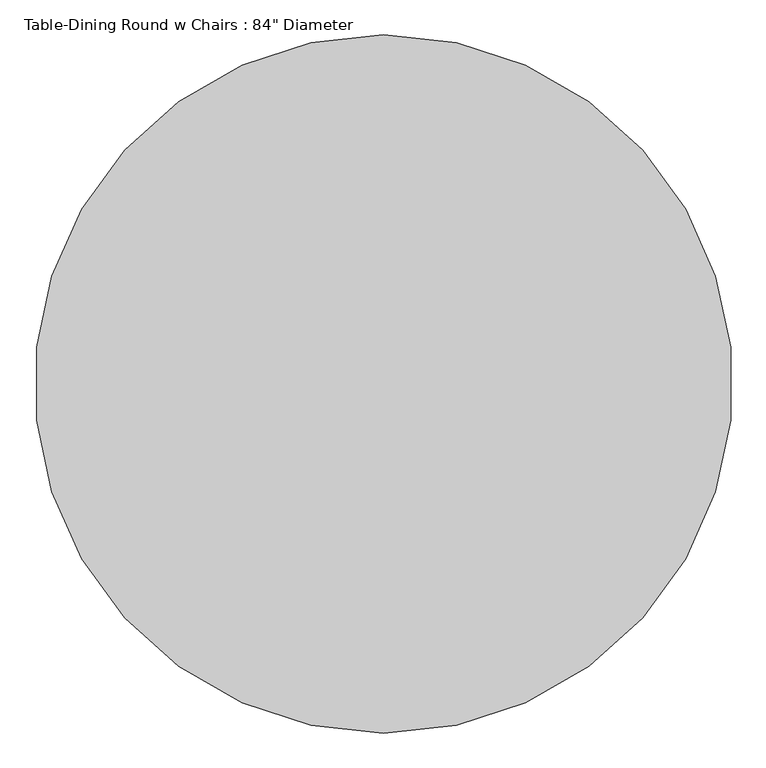
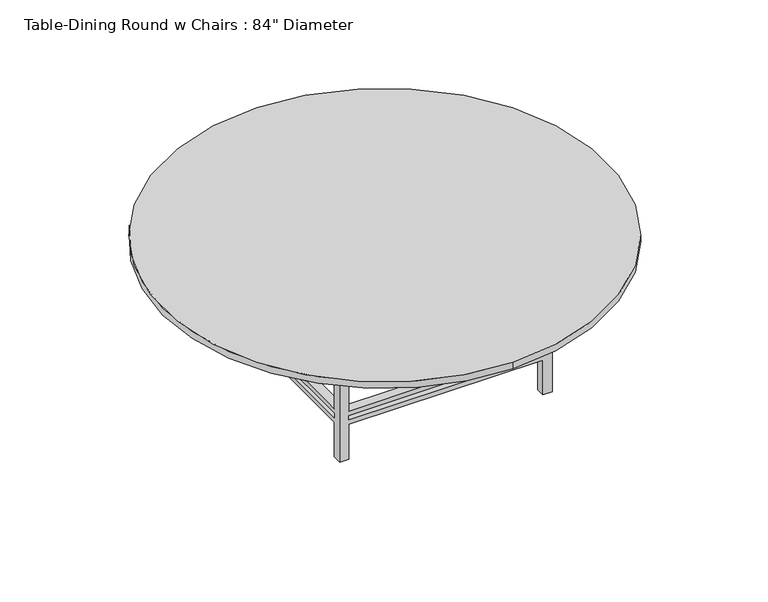
"""IFC4 building model written with IfcOpenShell, lengths in millimetres: furniture geometry."""

from ifc_helpers import new_model, si_unit, point, frame, frame_2d, origin, place, context, project, spatial, polyline, circle_curve, trimmed, segment, composite_curve, outline, extrude, faceted_brep, source, transform, mapped, element, save


def furniture_9698bf4d(model_context):
    return source(origin(), model_context, "Body", "SolidModel", [
        extrude(outline(polyline([(713.2819672, 424.7213115), (713.2819672, -794.4786885), (-505.9180328, -794.4786885), (-505.9180328, 424.7213115), (713.2819672, 424.7213115)]), holes=[polyline([(687.8819672, 399.3213115), (-480.5180328, 399.3213115), (-480.5180328, -769.0786885), (687.8819672, -769.0786885), (687.8819672, 399.3213115)])]), frame((0.0, 0.0, 647.7), z_axis=(0.0, 0.0, 1.0), x_axis=(1.0, 0.0, 0.0)), (0.0, 0.0, 1.0), 76.2),
        faceted_brep([(637.0819672, 348.5213115, 279.4), (637.0819672, -718.2786885, 279.4), (687.8819672, -718.2786885, 279.4), (687.8819672, 348.5213115, 279.4), (-429.7180328, -718.2786885, 279.4), (-429.7180328, -769.0786885, 279.4), (637.0819672, -769.0786885, 279.4), (-429.7180328, 348.5213115, 279.4), (-480.5180328, 348.5213115, 279.4), (-480.5180328, -718.2786885, 279.4), (637.0819672, 399.3213115, 279.4), (-429.7180328, 399.3213115, 279.4), (637.0819672, 348.5213115, 254.0), (-429.7180328, 348.5213115, 254.0), (-429.7180328, 399.3213115, 254.0), (637.0819672, 399.3213115, 254.0), (-429.7180328, -718.2786885, 254.0), (-480.5180328, -718.2786885, 254.0), (-480.5180328, 348.5213115, 254.0), (637.0819672, -718.2786885, 254.0), (637.0819672, -769.0786885, 254.0), (-429.7180328, -769.0786885, 254.0), (687.8819672, 348.5213115, 254.0), (687.8819672, -718.2786885, 254.0), (-480.5180328, 399.3213115, 647.7), (-429.7180328, 399.3213115, 647.7), (637.0819672, 399.3213115, 647.7), (687.8819672, 399.3213115, 647.7), (687.8819672, 399.3213115, 0.0), (637.0819672, 399.3213115, 0.0), (637.0819672, 399.3213115, 203.2), (-429.7180328, 399.3213115, 203.2), (-429.7180328, 399.3213115, 0.0), (-480.5180328, 399.3213115, 0.0), (-429.7180328, 399.3213115, 228.6), (637.0819672, 399.3213115, 228.6), (-480.5180328, 348.5213115, 647.7), (-480.5180328, 348.5213115, 0.0), (-480.5180328, 348.5213115, 203.2), (-480.5180328, -718.2786885, 203.2), (-480.5180328, -718.2786885, 0.0), (-480.5180328, -769.0786885, 0.0), (-480.5180328, -769.0786885, 647.7), (-480.5180328, -718.2786885, 647.7), (-480.5180328, -718.2786885, 228.6), (-480.5180328, 348.5213115, 228.6), (687.8819672, -769.0786885, 647.7), (637.0819672, -769.0786885, 647.7), (-429.7180328, -769.0786885, 647.7), (-429.7180328, -769.0786885, 0.0), (-429.7180328, -769.0786885, 203.2), (637.0819672, -769.0786885, 203.2), (637.0819672, -769.0786885, 0.0), (687.8819672, -769.0786885, 0.0), (637.0819672, -769.0786885, 228.6), (-429.7180328, -769.0786885, 228.6), (687.8819672, 348.5213115, 647.7), (687.8819672, -718.2786885, 647.7), (687.8819672, -718.2786885, 0.0), (687.8819672, -718.2786885, 203.2), (687.8819672, 348.5213115, 203.2), (687.8819672, 348.5213115, 0.0), (687.8819672, 348.5213115, 228.6), (687.8819672, -718.2786885, 228.6), (-429.7180328, 348.5213115, 647.7), (637.0819672, -718.2786885, 647.7), (637.0819672, 348.5213115, 647.7), (-429.7180328, -718.2786885, 647.7), (637.0819672, 348.5213115, 0.0), (-429.7180328, -718.2786885, 0.0), (-429.7180328, 348.5213115, 0.0), (637.0819672, -718.2786885, 0.0), (-429.7180328, 348.5213115, 228.6), (-429.7180328, 348.5213115, 203.2), (637.0819672, 348.5213115, 228.6), (637.0819672, 348.5213115, 203.2), (637.0819672, -718.2786885, 228.6), (637.0819672, -718.2786885, 203.2), (-429.7180328, -718.2786885, 228.6), (-429.7180328, -718.2786885, 203.2)], [[[0, 1, 2, 3]], [[1, 4, 5, 6]], [[4, 7, 8, 9]], [[7, 0, 10, 11]], [[12, 13, 14, 15]], [[13, 16, 17, 18]], [[16, 19, 20, 21]], [[19, 12, 22, 23]], [[24, 25, 11, 10, 26, 27, 28, 29, 30, 31, 32, 33], [14, 34, 35, 15]], [[36, 24, 33, 37, 38, 39, 40, 41, 42, 43, 9, 8], [17, 44, 45, 18]], [[46, 47, 6, 5, 48, 42, 41, 49, 50, 51, 52, 53], [20, 54, 55, 21]], [[28, 27, 56, 3, 2, 57, 46, 53, 58, 59, 60, 61], [22, 62, 63, 23]], [[1, 0, 12, 19]], [[4, 1, 19, 16]], [[7, 4, 16, 13]], [[0, 7, 13, 12]], [[25, 24, 36, 64]], [[47, 46, 57, 65]], [[26, 66, 56, 27]], [[48, 67, 43, 42]], [[29, 28, 61, 68]], [[49, 41, 40, 69]], [[32, 70, 37, 33]], [[52, 71, 58, 53]], [[13, 18, 45, 72]], [[64, 36, 8, 7]], [[37, 70, 73, 38]], [[14, 13, 72, 34]], [[25, 64, 7, 11]], [[70, 32, 31, 73]], [[12, 15, 35, 74]], [[66, 26, 10, 0]], [[29, 68, 75, 30]], [[22, 12, 74, 62]], [[56, 66, 0, 3]], [[68, 61, 60, 75]], [[19, 23, 63, 76]], [[65, 57, 2, 1]], [[58, 71, 77, 59]], [[20, 19, 76, 54]], [[47, 65, 1, 6]], [[71, 52, 51, 77]], [[16, 21, 55, 78]], [[67, 48, 5, 4]], [[49, 69, 79, 50]], [[17, 16, 78, 44]], [[43, 67, 4, 9]], [[69, 40, 39, 79]], [[74, 76, 63, 62]], [[76, 78, 55, 54]], [[78, 72, 45, 44]], [[72, 74, 35, 34]], [[75, 73, 31, 30]], [[73, 79, 39, 38]], [[79, 77, 51, 50]], [[77, 75, 60, 59]], [[76, 74, 75, 77]], [[78, 76, 77, 79]], [[72, 78, 79, 73]], [[74, 72, 73, 75]]]),
        extrude(outline(composite_curve([segment(trimmed(circle_curve(frame_2d((103.6819672, -184.8786885)), 1219.2), [point((103.6819672, -1404.0786885))], [point((103.6819672, 1034.3213115))], False, "CARTESIAN"), True, "CONTINUOUS"), segment(trimmed(circle_curve(frame_2d((103.6819672, -184.8786885)), 1219.2), [point((103.6819672, 1034.3213115))], [point((103.6819672, -1404.0786885))], False, "CARTESIAN"), True, "CONTINUOUS")], self_intersect=False)), frame((0.0, 0.0, 723.9), z_axis=(0.0, 0.0, 1.0), x_axis=(1.0, 0.0, 0.0)), (0.0, 0.0, 1.0), 38.1),
    ])


if __name__ == "__main__":
    model = new_model("IFC4")
    model_context = context("Model", 3, world=origin())
    ifc_project = project(units=[si_unit("LENGTHUNIT", "METRE", prefix="MILLI")], contexts=[model_context])
    site = spatial("IfcSite", under=ifc_project)
    building = spatial("IfcBuilding", under=site)
    placement = place(None, origin())
    furniture_shape = furniture_9698bf4d(model_context)
    element("IfcFurniture", 1, ObjectType="Table-Dining Round w Chairs : 84\" Diameter", at=placement, inside=building, context=model_context, shape_type="MappedRepresentation", body=[
        mapped(furniture_shape, transform((0.0, 0.0, 0.0), x_axis=(1.0, 0.0, 0.0), y_axis=(0.0, 1.0, 0.0), z_axis=(0.0, 0.0, 1.0))),
    ])
    save(model, "model.ifc")

# Revit data of these elements
# Type "Table-Dining Round w Chairs : 84\" Diameter"
#   Assembly Code = "E2020200"
#   Radius = 4' - 0"
#   Diameter = 8' - 0"
#   Height = 2' - 6"
#   Chairs = 10
#   Base Material = Pine
#   Top Material = Laminate, Linen, Matte
#   Default Elevation = 0
# Element 1 (IfcFurniture, "Table-Dining Round w Chairs : 84\" Diameter")
#   Materials on its faces: "Pine", "Laminate, Linen, Matte"
# Materials
#   "Pine": class "Wood", colour RGB 234 198 147, transparency 0, Description = "Pinus Echinata", Cost = 0
#   "Laminate, Linen, Matte": class "Plastic", colour RGB 198 189 176, transparency 0, Description = "Plastic Laminate - Linen, Matte", Cost = 0
